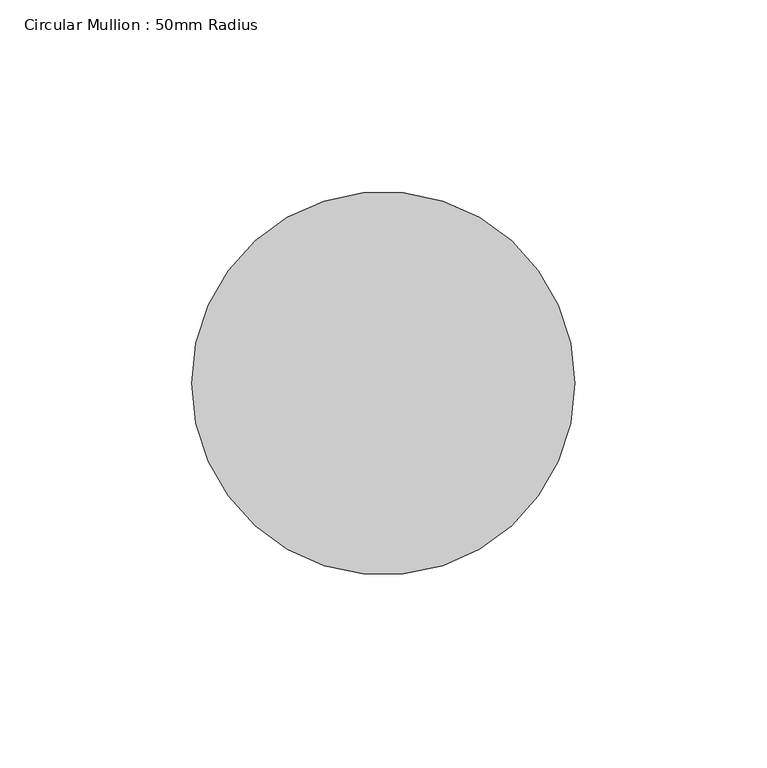
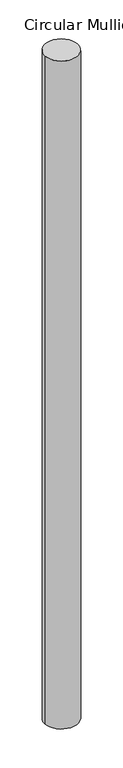
"""IFC4 building model written with IfcOpenShell, lengths in millimetres: member geometry, Circular Mullion : 50mm Radius."""

from ifc_helpers import new_model, si_unit, point, frame, origin, origin_2d, place, context, project, spatial, circle_curve, trimmed, segment, composite_curve, outline, extrude, source, transform, mapped, element, save


def circular_mullion_50mm_radius_93405507(model_context):
    return source(origin(), model_context, "Body", "SweptSolid", [
        extrude(outline(composite_curve([segment(trimmed(circle_curve(origin_2d(), 50.0), [point((50.0, 0.0))], [point((-50.0, 0.0))], False, "CARTESIAN"), True, "CONTINUOUS"), segment(trimmed(circle_curve(origin_2d(), 50.0), [point((-50.0, 0.0))], [point((50.0, 0.0))], False, "CARTESIAN"), True, "CONTINUOUS")], self_intersect=False)), frame((0.0, 0.0, -2112.4596552), z_axis=(0.0, 0.0, 1.0), x_axis=(1.0, 0.0, 0.0)), (0.0, 0.0, 1.0), 2112.4596552),
    ])


if __name__ == "__main__":
    model = new_model("IFC4")
    model_context = context("Model", 3, world=origin())
    ifc_project = project(units=[si_unit("LENGTHUNIT", "METRE", prefix="MILLI")], contexts=[model_context])
    site = spatial("IfcSite", under=ifc_project)
    building = spatial("IfcBuilding", under=site)
    placement = place(None, origin())
    circular_mullion_50mm_radius_shape = circular_mullion_50mm_radius_93405507(model_context)
    element("IfcMember", 1, ObjectType="Circular Mullion : 50mm Radius", at=placement, inside=building, context=model_context, shape_type="MappedRepresentation", body=[
        mapped(circular_mullion_50mm_radius_shape, transform((0.0, 0.0, 0.0), x_axis=(1.0, 0.0, 0.0), y_axis=(0.0, 1.0, 0.0), z_axis=(0.0, 0.0, 1.0))),
    ])
    save(model, "model.ifc")

# Revit data of these elements
# Type "Circular Mullion : 50mm Radius"
#   built-in parameter 1007350 = 0.164042 (stored number, unit not read)
# Element 1 (IfcMember, "Circular Mullion : 50mm Radius")
#   Materials on its faces: "Aluminium"
# Materials
#   "Aluminium": class "Metal", colour RGB 247 247 247, transparency 0, Description = "Aluminium 6061", Cost = 0
